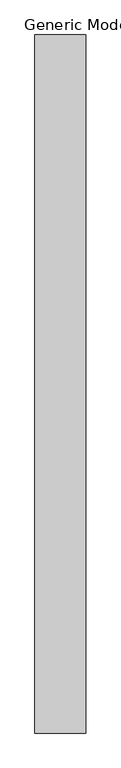
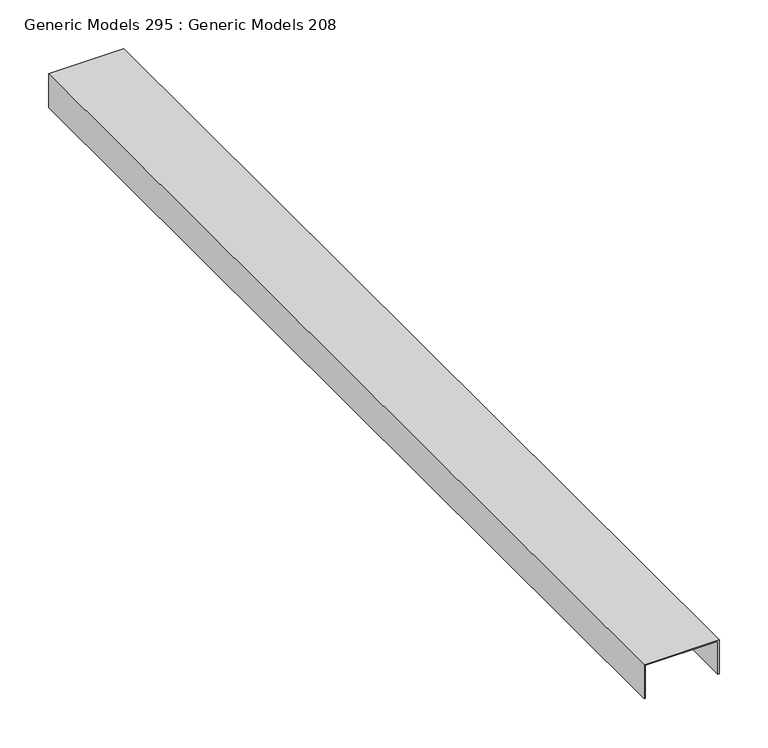
"""IFC4 building model written with IfcOpenShell, lengths in millimetres: proxy geometry, Generic Models 295 : Generic Models 208."""

from ifc_helpers import new_model, si_unit, frame, origin, place, context, project, spatial, polyline, outline, extrude, source, transform, mapped, element, save


def generic_models_295_generic_models_208_65722f1e(model_context):
    return source(origin(), model_context, "Body", "SweptSolid", [
        extrude(outline(polyline([(2037.953125, 55683.9204676), (2079.228125, 55683.9204676), (2079.228125, 55769.6454676), (2037.953125, 55769.6454676), (2037.953125, 55771.2329676), (2080.815625, 55771.2329676), (2080.815625, 55682.3329676), (2037.953125, 55682.3329676), (2037.953125, 55683.9204676)])), frame((0.0, -228.7033818, 0.0), z_axis=(0.0, 1.0, 0.0), x_axis=(0.0, 0.0, 1.0)), (0.0, 0.0, 1.0), 1219.2),
    ])


if __name__ == "__main__":
    model = new_model("IFC4")
    model_context = context("Model", 3, world=origin())
    ifc_project = project(units=[si_unit("LENGTHUNIT", "METRE", prefix="MILLI")], contexts=[model_context])
    site = spatial("IfcSite", under=ifc_project)
    building = spatial("IfcBuilding", under=site)
    placement = place(None, origin())
    generic_models_295_generic_models_208_shape = generic_models_295_generic_models_208_65722f1e(model_context)
    element("IfcBuildingElementProxy", 1, Name="Generic Models 295 : Generic Models 208", ObjectType="Generic Models 295 : Generic Models 208", at=placement, inside=building, context=model_context, shape_type="MappedRepresentation", body=[
        mapped(generic_models_295_generic_models_208_shape, transform((0.0, 0.0, 0.0), x_axis=(1.0, 0.0, 0.0), y_axis=(0.0, 1.0, 0.0), z_axis=(0.0, 0.0, 1.0))),
    ])
    save(model, "model.ifc")

# Revit data of these elements
# Element 1 (IfcBuildingElementProxy, "Generic Models 295 : Generic Models 208")
#   Materials on its faces: "METAL STUD CAP"
# Materials
#   "METAL STUD CAP": class "Metal", colour RGB 244 244 244, transparency 0, Description = "Aluminum 6061", Cost = 0
